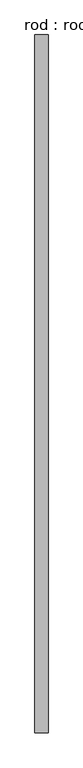
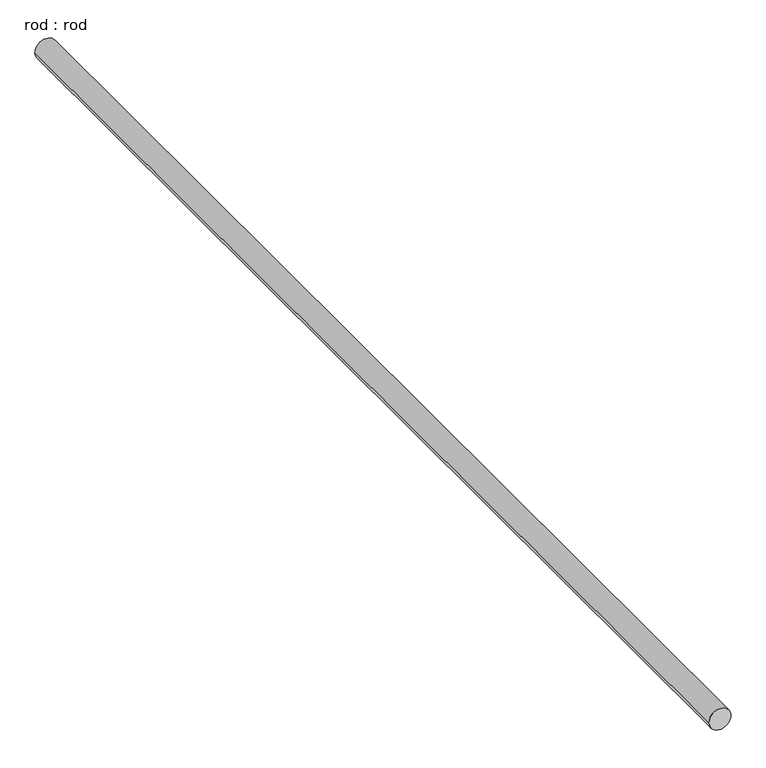
"""IFC4 building model written with IfcOpenShell, lengths in millimetres: proxy geometry, rod : rod."""

from ifc_helpers import new_model, si_unit, point, frame, frame_2d, origin, place, context, project, spatial, circle_curve, trimmed, segment, composite_curve, outline, extrude, source, transform, mapped, element, save


def rod_rod_51a05636(model_context):
    return source(origin(), model_context, "Body", "SweptSolid", [
        extrude(outline(composite_curve([segment(trimmed(circle_curve(frame_2d((0.0108462, 0.0)), 200.0), [point((0.0108462, 200.0))], [point((0.0108462, -200.0))], False, "CARTESIAN"), True, "CONTINUOUS"), segment(trimmed(circle_curve(frame_2d((0.0108462, 0.0)), 200.0), [point((0.0108462, -200.0))], [point((0.0108462, 200.0))], False, "CARTESIAN"), True, "CONTINUOUS")], self_intersect=False)), frame((0.0, -6502.1404259, 0.0), z_axis=(0.0, 1.0, 0.0), x_axis=(0.0, 0.0, 1.0)), (0.0, 0.0, 1.0), 21189.7380824),
    ])


if __name__ == "__main__":
    model = new_model("IFC4")
    model_context = context("Model", 3, world=origin())
    ifc_project = project(units=[si_unit("LENGTHUNIT", "METRE", prefix="MILLI")], contexts=[model_context])
    site = spatial("IfcSite", under=ifc_project)
    building = spatial("IfcBuilding", under=site)
    placement = place(None, origin())
    rod_rod_shape = rod_rod_51a05636(model_context)
    element("IfcBuildingElementProxy", 1, Name="rod : rod", ObjectType="rod : rod", at=placement, inside=building, context=model_context, shape_type="MappedRepresentation", body=[
        mapped(rod_rod_shape, transform((0.0, 0.0, 0.0), x_axis=(1.0, 0.0, 0.0), y_axis=(0.0, 1.0, 0.0), z_axis=(0.0, 0.0, 1.0))),
    ])
    save(model, "model.ifc")

# Revit data of these elements
# Type "rod : rod"
#   Default Elevation = 0
